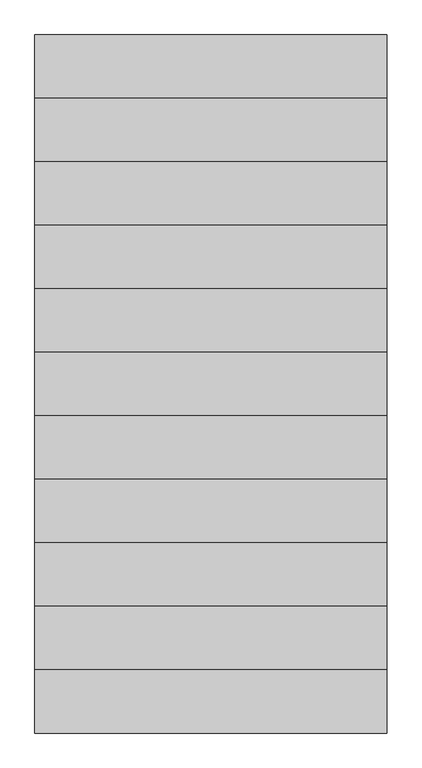
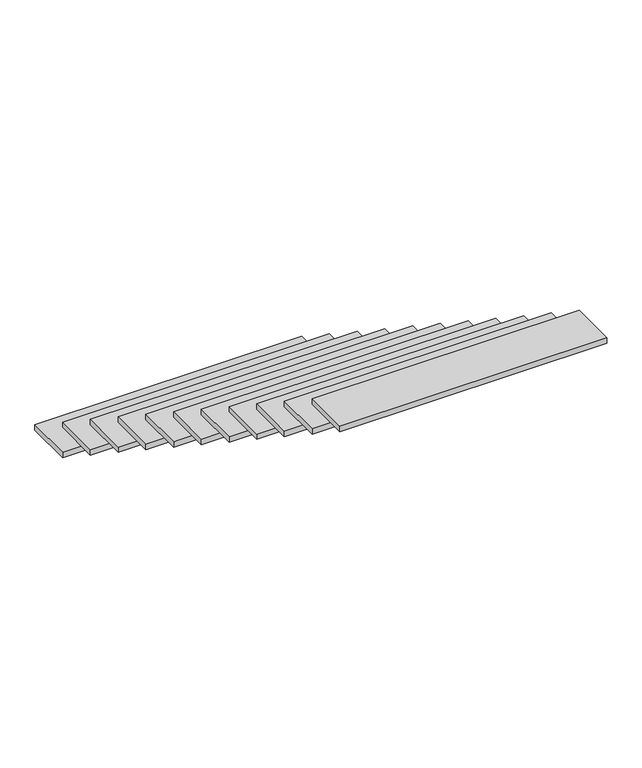
"""IFC4 building model written with IfcOpenShell, lengths in millimetres: stair flight geometry."""

import ifcopenshell
import ifcopenshell.guid

model = None  # the IFC model being written
_history = None  # IfcOwnerHistory: only IFC2X3 demands one
_inside = {}  # id of a spatial element -> (the spatial element, [elements in it])
_under = {}  # id of a project, library or spatial element -> (it, [spatial elements below it])
_declared = {}  # id of a project -> (the project, [libraries it declares])
_typed = {}  # id of a type object -> (the type object, [elements of that type])
_made_of = {}  # id of a material, layer set ... -> (it, [elements and type objects made of it])


def new_model(schema):
    """Start an empty IFC model of exactly this schema.

    Asked for "IFC4X3", IfcOpenShell would pick the latest addendum, in which some entities
    have other attributes; the version numbers below select the first issue.
    IFC2X3 requires an IfcOwnerHistory on every rooted entity: one is made here for all.
    """
    global model, _history
    if schema == "IFC4X3":
        model = ifcopenshell.file(schema_version=(4, 3, 0, 0))
    else:
        model = ifcopenshell.file(schema=schema)
    _inside.clear()
    _under.clear()
    _declared.clear()
    _typed.clear()
    _made_of.clear()
    _history = None
    if model.schema == "IFC2X3":
        org = make("IfcOrganization", Name="unknown")
        user = make(
            "IfcPersonAndOrganization",
            ThePerson=make("IfcPerson", FamilyName="unknown"),
            TheOrganization=org,
        )
        app = make(
            "IfcApplication",
            ApplicationDeveloper=org,
            Version="unknown",
            ApplicationFullName="unknown",
            ApplicationIdentifier="unknown",
        )
        _history = make(
            "IfcOwnerHistory",
            OwningUser=user,
            OwningApplication=app,
            ChangeAction="ADDED",
            CreationDate=0,
        )
    return model


def make(cls, **values):
    """One entity of the class cls with the attributes given. An attribute that is None is left unset."""
    return model.create_entity(
        cls, **{name: value for name, value in values.items() if value is not None}
    )


def rooted(cls, **values):
    """An entity with a GlobalId (a new one), such as an element, a storey or a relation."""
    return make(cls, GlobalId=ifcopenshell.guid.new(), OwnerHistory=_history, **values)


def si_unit(unit_type, name, prefix=None):
    """IfcSIUnit, for example si_unit("LENGTHUNIT", "METRE", prefix="MILLI")."""
    return make("IfcSIUnit", UnitType=unit_type, Prefix=prefix, Name=name)


def assignment(units):
    """IfcUnitAssignment: the units of a project."""
    return None if units is None else make("IfcUnitAssignment", Units=units)


def point(xyz):
    """IfcCartesianPoint."""
    return None if xyz is None else make("IfcCartesianPoint", Coordinates=xyz)


def direction(xyz):
    """IfcDirection."""
    return None if xyz is None else make("IfcDirection", DirectionRatios=xyz)


def frame(location, z_axis=None, x_axis=None):
    """IfcAxis2Placement3D, a coordinate frame: its origin and axes. An axis left out is left unset."""
    return make(
        "IfcAxis2Placement3D",
        Location=point(location),
        Axis=direction(z_axis),
        RefDirection=direction(x_axis),
    )


def origin():
    """The frame at (0, 0, 0) with its axes left unset."""
    return frame((0.0, 0.0, 0.0))


def place(relative_to, where):
    """IfcLocalPlacement: puts the frame where relative to a parent placement (None: the world)."""
    return make(
        "IfcLocalPlacement", PlacementRelTo=relative_to, RelativePlacement=where
    )


def context(
    kind, dimensions, precision=None, world=None, true_north=None, identifier=None
):
    """IfcGeometricRepresentationContext, for example the 3D "Model" context."""
    return make(
        "IfcGeometricRepresentationContext",
        ContextIdentifier=identifier,
        ContextType=kind,
        CoordinateSpaceDimension=dimensions,
        Precision=precision,
        WorldCoordinateSystem=world,
        TrueNorth=true_north,
    )


def project(units=None, contexts=None):
    """IfcProject with its units and contexts."""
    return rooted(
        "IfcProject",
        Name="project",
        RepresentationContexts=contexts,
        UnitsInContext=assignment(units),
    )


def spatial(cls, under=None, at=None, **own):
    """A site, building, storey or space (cls), placed at a placement, below another one or the project."""
    s = rooted(cls, ObjectPlacement=at, **own)
    if under is not None:
        _under.setdefault(under.id(), (under, []))[1].append(s)
    return s


def polyline(points):
    """IfcPolyline through the points."""
    return make("IfcPolyline", Points=[point(p) for p in points])


def outline(outer, holes=None, kind="AREA"):
    """IfcArbitraryClosedProfileDef: a profile drawn as a closed curve; with holes, ...WithVoids."""
    if holes is None:
        return make("IfcArbitraryClosedProfileDef", ProfileType=kind, OuterCurve=outer)
    return make(
        "IfcArbitraryProfileDefWithVoids",
        ProfileType=kind,
        OuterCurve=outer,
        InnerCurves=holes,
    )


def extrude(swept, where, along, depth):
    """IfcExtrudedAreaSolid: the profile swept, set in the frame where, extruded along a direction by depth."""
    return make(
        "IfcExtrudedAreaSolid",
        SweptArea=swept,
        Position=where,
        ExtrudedDirection=direction(along),
        Depth=depth,
    )


def shape(context_of_items, identifier, shape_type, items):
    """IfcShapeRepresentation: the items that make up one representation, for example the "Body"."""
    return make(
        "IfcShapeRepresentation",
        ContextOfItems=context_of_items,
        RepresentationIdentifier=identifier,
        RepresentationType=shape_type,
        Items=items,
    )


def source(mapping_origin, context_of_items, identifier, shape_type, items):
    """IfcRepresentationMap: a shape defined once, which mapped items show again and again."""
    return make(
        "IfcRepresentationMap",
        MappingOrigin=mapping_origin,
        MappedRepresentation=shape(context_of_items, identifier, shape_type, items),
    )


def transform(
    local_origin,
    x_axis=None,
    y_axis=None,
    z_axis=None,
    scale=None,
    scale2=None,
    scale3=None,
    uniform=True,
):
    """IfcCartesianTransformationOperator3D, or its non-uniform kind. x_axis, y_axis, z_axis: its Axis1, 2, 3."""
    if uniform:
        return make(
            "IfcCartesianTransformationOperator3D",
            Axis1=direction(x_axis),
            Axis2=direction(y_axis),
            LocalOrigin=point(local_origin),
            Scale=scale,
            Axis3=direction(z_axis),
        )
    return make(
        "IfcCartesianTransformationOperator3DnonUniform",
        Axis1=direction(x_axis),
        Axis2=direction(y_axis),
        LocalOrigin=point(local_origin),
        Scale=scale,
        Axis3=direction(z_axis),
        Scale2=scale2,
        Scale3=scale3,
    )


def mapped(mapping_source, mapping_target):
    """IfcMappedItem: shows the shape of a source again, moved by a transform."""
    return make(
        "IfcMappedItem", MappingSource=mapping_source, MappingTarget=mapping_target
    )


def made_of(thing, what):
    """Note that an element or type object is made of a material, layer set ...; save() writes the relation."""
    if what is not None:
        _made_of.setdefault(what.id(), (what, []))[1].append(thing)
    return thing


def element(
    cls,
    number,
    at=None,
    inside=None,
    cuts=None,
    type_object=None,
    material=None,
    context=None,
    identifier="Body",
    shape_type=None,
    held_by="IfcProductDefinitionShape",
    body=None,
    shapes=None,
    **own,
):
    """One element of the class cls, such as IfcWall. Its Tag is "e" and its number.

    at: its placement. inside: the storey or other place that contains it. cuts: it is an
    opening in that element (IfcRelVoidsElement). A single representation is given by context,
    identifier, shape_type and body (its items); several are given by shapes. held_by: the class
    of the entity that holds the representations. save() writes the other relations.
    """
    e = rooted(cls, Tag="e%d" % number, ObjectPlacement=at, **own)
    if body is not None:
        shapes = [shape(context, identifier, shape_type, body)]
    if shapes is not None:
        e.Representation = make(held_by, Representations=shapes)
    if inside is not None:
        _inside.setdefault(inside.id(), (inside, []))[1].append(e)
    if cuts is not None:
        rooted(
            "IfcRelVoidsElement", RelatingBuildingElement=cuts, RelatedOpeningElement=e
        )
    if type_object is not None:
        _typed.setdefault(type_object.id(), (type_object, []))[1].append(e)
    return made_of(e, material)


def aggregate(whole, parts):
    """IfcRelAggregates: a whole, such as a stair, and the parts it consists of."""
    return rooted("IfcRelAggregates", RelatingObject=whole, RelatedObjects=parts)


def save(model, path):
    """Write the relations noted so far, then the file.

    IfcRelAggregates (storeys below a building ...), IfcRelContainedInSpatialStructure (elements
    in a storey), IfcRelDefinesByType, IfcRelAssociatesMaterial and IfcRelDeclares: one each for
    every whole, place, type object, material and project.
    """
    for whole, parts in _under.values():
        aggregate(whole, parts)
    for where, things in _inside.values():
        rooted(
            "IfcRelContainedInSpatialStructure",
            RelatedElements=things,
            RelatingStructure=where,
        )
    for kind, things in _typed.values():
        rooted("IfcRelDefinesByType", RelatedObjects=things, RelatingType=kind)
    for what, things in _made_of.values():
        rooted("IfcRelAssociatesMaterial", RelatedObjects=things, RelatingMaterial=what)
    for by, libraries in _declared.values():
        rooted("IfcRelDeclares", RelatingContext=by, RelatedDefinitions=libraries)
    model.write(path)


def stair_flight_7c2b7268(model_context):
    return source(origin(), model_context, "Body", "SweptSolid", [
        extrude(outline(polyline([(16085.3403387, 4647.6066446), (14585.3403387, 4647.6066446), (14585.3403387, 4917.6066446), (16085.3403387, 4917.6066446), (16085.3403387, 4647.6066446)])), frame((0.0, 0.0, 13939.4285714), z_axis=(0.0, 0.0, 1.0), x_axis=(1.0, 0.0, 0.0)), (0.0, 0.0, 1.0), 32.0),
        extrude(outline(polyline([(16085.3403387, 4377.6066446), (14585.3403387, 4377.6066446), (14585.3403387, 4647.6066446), (16085.3403387, 4647.6066446), (16085.3403387, 4377.6066446)])), frame((0.0, 0.0, 14118.5494505), z_axis=(0.0, 0.0, 1.0), x_axis=(1.0, 0.0, 0.0)), (0.0, 0.0, 1.0), 32.0),
        extrude(outline(polyline([(16085.3403387, 4107.6066446), (14585.3403387, 4107.6066446), (14585.3403387, 4377.6066446), (16085.3403387, 4377.6066446), (16085.3403387, 4107.6066446)])), frame((0.0, 0.0, 14297.6703297), z_axis=(0.0, 0.0, 1.0), x_axis=(1.0, 0.0, 0.0)), (0.0, 0.0, 1.0), 32.0),
        extrude(outline(polyline([(16085.3403387, 3837.6066446), (14585.3403387, 3837.6066446), (14585.3403387, 4107.6066446), (16085.3403387, 4107.6066446), (16085.3403387, 3837.6066446)])), frame((0.0, 0.0, 14476.7912088), z_axis=(0.0, 0.0, 1.0), x_axis=(1.0, 0.0, 0.0)), (0.0, 0.0, 1.0), 32.0),
        extrude(outline(polyline([(16085.3403387, 3567.6066446), (14585.3403387, 3567.6066446), (14585.3403387, 3837.6066446), (16085.3403387, 3837.6066446), (16085.3403387, 3567.6066446)])), frame((0.0, 0.0, 14655.9120879), z_axis=(0.0, 0.0, 1.0), x_axis=(1.0, 0.0, 0.0)), (0.0, 0.0, 1.0), 32.0),
        extrude(outline(polyline([(16085.3403387, 3297.6066446), (14585.3403387, 3297.6066446), (14585.3403387, 3567.6066446), (16085.3403387, 3567.6066446), (16085.3403387, 3297.6066446)])), frame((0.0, 0.0, 14835.032967), z_axis=(0.0, 0.0, 1.0), x_axis=(1.0, 0.0, 0.0)), (0.0, 0.0, 1.0), 32.0),
        extrude(outline(polyline([(16085.3403387, 3027.6066446), (14585.3403387, 3027.6066446), (14585.3403387, 3297.6066446), (16085.3403387, 3297.6066446), (16085.3403387, 3027.6066446)])), frame((0.0, 0.0, 15014.1538462), z_axis=(0.0, 0.0, 1.0), x_axis=(1.0, 0.0, 0.0)), (0.0, 0.0, 1.0), 32.0),
        extrude(outline(polyline([(16085.3403387, 2757.6066446), (14585.3403387, 2757.6066446), (14585.3403387, 3027.6066446), (16085.3403387, 3027.6066446), (16085.3403387, 2757.6066446)])), frame((0.0, 0.0, 15193.2747253), z_axis=(0.0, 0.0, 1.0), x_axis=(1.0, 0.0, 0.0)), (0.0, 0.0, 1.0), 32.0),
        extrude(outline(polyline([(16085.3403387, 2487.6066446), (14585.3403387, 2487.6066446), (14585.3403387, 2757.6066446), (16085.3403387, 2757.6066446), (16085.3403387, 2487.6066446)])), frame((0.0, 0.0, 15372.3956044), z_axis=(0.0, 0.0, 1.0), x_axis=(1.0, 0.0, 0.0)), (0.0, 0.0, 1.0), 32.0),
        extrude(outline(polyline([(16085.3403387, 2217.6066446), (14585.3403387, 2217.6066446), (14585.3403387, 2487.6066446), (16085.3403387, 2487.6066446), (16085.3403387, 2217.6066446)])), frame((0.0, 0.0, 15551.5164835), z_axis=(0.0, 0.0, 1.0), x_axis=(1.0, 0.0, 0.0)), (0.0, 0.0, 1.0), 32.0),
        extrude(outline(polyline([(16085.3403387, 1947.6066446), (14585.3403387, 1947.6066446), (14585.3403387, 2217.6066446), (16085.3403387, 2217.6066446), (16085.3403387, 1947.6066446)])), frame((0.0, 0.0, 15730.6373626), z_axis=(0.0, 0.0, 1.0), x_axis=(1.0, 0.0, 0.0)), (0.0, 0.0, 1.0), 32.0),
    ])


if __name__ == "__main__":
    model = new_model("IFC4")
    model_context = context("Model", 3, world=origin())
    ifc_project = project(units=[si_unit("LENGTHUNIT", "METRE", prefix="MILLI")], contexts=[model_context])
    site = spatial("IfcSite", under=ifc_project)
    building = spatial("IfcBuilding", under=site)
    placement = place(None, origin())
    stair_flight_shape = stair_flight_7c2b7268(model_context)
    element("IfcStairFlight", 1, at=placement, inside=building, context=model_context, shape_type="MappedRepresentation", body=[
        mapped(stair_flight_shape, transform((0.0, 0.0, 0.0), x_axis=(1.0, 0.0, 0.0), y_axis=(0.0, 1.0, 0.0), z_axis=(0.0, 0.0, 1.0))),
    ])
    save(model, "model.ifc")

# Revit data of these elements
# Element 1 (IfcStairFlight)
#   Materials on its faces: "철강"
# Materials
#   "철강": class "Generic", colour RGB 143 142 141, transparency 0, Description = "철골+가공조립+세우기", Cost = 0
